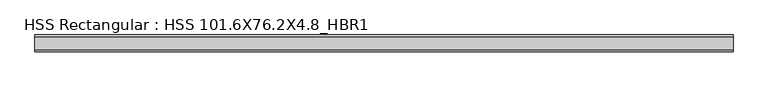
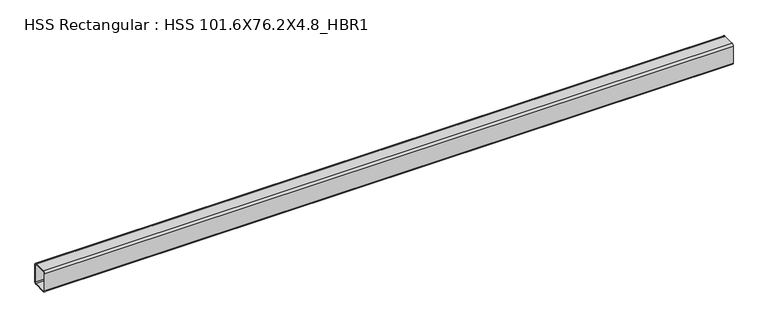
"""IFC4 building model written with IfcOpenShell, lengths in millimetres: beam geometry, HSS Rectangular : HSS 101.6X76.2X4.8_HBR1."""

from ifc_helpers import new_model, si_unit, point, frame, frame_2d, origin, place, context, project, spatial, polyline, circle_curve, trimmed, segment, composite_curve, outline, extrude, source, transform, mapped, element, save


def hss_rectangular_hss_101_6x76_2x4_8_hbr1_8cfbb8c3(model_context):
    return source(origin(), model_context, "Body", "SweptSolid", [
        extrude(outline(composite_curve([segment(polyline([(38.1, 41.275), (38.1, -41.275)]), True, "CONTINUOUS"), segment(trimmed(circle_curve(frame_2d((28.575, -41.275)), 9.525), [point((38.1, -41.275))], [point((28.575, -50.8))], False, "CARTESIAN"), True, "CONTINUOUS"), segment(polyline([(28.575, -50.8), (-28.575, -50.8)]), True, "CONTINUOUS"), segment(trimmed(circle_curve(frame_2d((-28.575, -41.275)), 9.525), [point((-28.575, -50.8))], [point((-38.1, -41.275))], False, "CARTESIAN"), True, "CONTINUOUS"), segment(polyline([(-38.1, -41.275), (-38.1, 41.275)]), True, "CONTINUOUS"), segment(trimmed(circle_curve(frame_2d((-28.575, 41.275)), 9.525), [point((-38.1, 41.275))], [point((-28.575, 50.8))], False, "CARTESIAN"), True, "CONTINUOUS"), segment(polyline([(-28.575, 50.8), (28.575, 50.8)]), True, "CONTINUOUS"), segment(trimmed(circle_curve(frame_2d((28.575, 41.275)), 9.525), [point((28.575, 50.8))], [point((38.1, 41.275))], False, "CARTESIAN"), True, "CONTINUOUS")], self_intersect=False), holes=[composite_curve([segment(trimmed(circle_curve(frame_2d((-28.575, 41.275)), 4.7625), [point((-28.575, 46.0375))], [point((-33.3375, 41.275))], True, "CARTESIAN"), True, "CONTINUOUS"), segment(polyline([(-33.3375, 41.275), (-33.3375, -41.275)]), True, "CONTINUOUS"), segment(trimmed(circle_curve(frame_2d((-28.575, -41.275)), 4.7625), [point((-33.3375, -41.275))], [point((-28.575, -46.0375))], True, "CARTESIAN"), True, "CONTINUOUS"), segment(polyline([(-28.575, -46.0375), (28.575, -46.0375)]), True, "CONTINUOUS"), segment(trimmed(circle_curve(frame_2d((28.575, -41.275)), 4.7625), [point((28.575, -46.0375))], [point((33.3375, -41.275))], True, "CARTESIAN"), True, "CONTINUOUS"), segment(polyline([(33.3375, -41.275), (33.3375, 41.275)]), True, "CONTINUOUS"), segment(trimmed(circle_curve(frame_2d((28.575, 41.275)), 4.7625), [point((33.3375, 41.275))], [point((28.575, 46.0375))], True, "CARTESIAN"), True, "CONTINUOUS"), segment(polyline([(28.575, 46.0375), (-28.575, 46.0375)]), True, "CONTINUOUS")], self_intersect=False)]), frame((-1609.0657472, 0.0, 0.0), z_axis=(1.0, 0.0, 0.0), x_axis=(0.0, 1.0, 0.0)), (0.0, 0.0, 1.0), 3182.7600999),
    ])


if __name__ == "__main__":
    model = new_model("IFC4")
    model_context = context("Model", 3, world=origin())
    ifc_project = project(units=[si_unit("LENGTHUNIT", "METRE", prefix="MILLI")], contexts=[model_context])
    site = spatial("IfcSite", under=ifc_project)
    building = spatial("IfcBuilding", under=site)
    placement = place(None, origin())
    hss_rectangular_hss_101_6x76_2x4_8_hbr1_shape = hss_rectangular_hss_101_6x76_2x4_8_hbr1_8cfbb8c3(model_context)
    element("IfcBeam", 1, ObjectType="HSS Rectangular : HSS 101.6X76.2X4.8_HBR1", at=placement, inside=building, context=model_context, shape_type="MappedRepresentation", body=[
        mapped(hss_rectangular_hss_101_6x76_2x4_8_hbr1_shape, transform((0.0, 0.0, 0.0), x_axis=(1.0, 0.0, 0.0), y_axis=(0.0, 1.0, 0.0), z_axis=(0.0, 0.0, 1.0))),
    ])
    save(model, "model.ifc")

# Revit data of these elements
# Type "HSS Rectangular : HSS 101.6X76.2X4.8_HBR1"
#   Section Name Key = "HSS 4X3X3/16"
#   Assembly Code = "B10"
#   Width = 7.62 cm
#   Wall Nominal Thickness = 0.4763 cm
#   Wall Design Thickness = 0.442 cm
#   Torsional Moment of Inertia = 260.561 cm⁴
#   Torsional Modulus = 61.2876 cm³
#   Section Area = 14.4516 cm²
#   Plastic Modulus weak axis = 40.3122 cm³
#   Plastic Modulus strong axis = 49.1612 cm³
#   Perimeter = 0.881482 m²/m
#   Outer Fillet = 0.9525 cm
#   Nominal Weight = 12.1285 kgf/m
#   Moment of Inertia weak axis = 131.529 cm⁴
#   Moment of Inertia strong axis = 205.202 cm⁴
#   Inner Fillet = 0.4763 cm
#   Height = 10.16 cm
#   Elastic Modulus weak axis = 34.4128 cm³
#   Elastic Modulus strong axis = 40.476 cm³
#   Centroid Vertical = 5.08 cm
#   Centroid Horizontal = 3.81 cm
#   Length [instance default] = 1524 mm
#   Structural Material [instance default] = Steel ASTM A500, Grade B, Rectangular and Square
#   Principal Axes Angle = 0
# Element 1 (IfcBeam, "HSS Rectangular : HSS 101.6X76.2X4.8_HBR1")
#   Structural Material = Steel ASTM A992
#   Materials on its faces: "Steel ASTM A992"
# Materials
#   "Steel ASTM A500, Grade B, Rectangular and Square": class "Metal", colour RGB 199 199 199, transparency 0, Description = "Carbon steel", Cost = 0
#   "Steel ASTM A992": class "Metal", colour RGB 199 199 199, transparency 0, Description = "Structural steel 50ksi", Cost = 0
